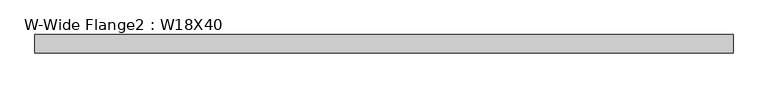
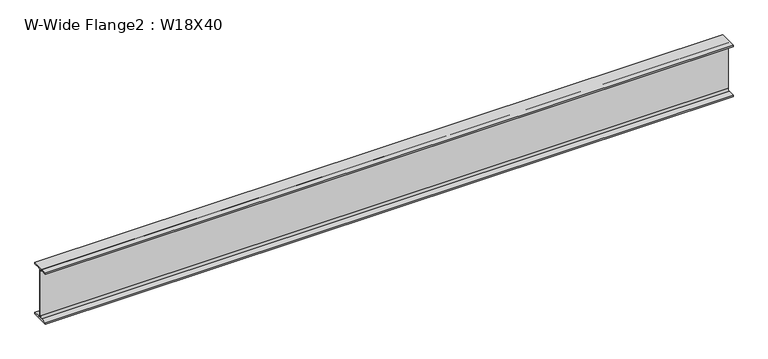
"""IFC4 building model written with IfcOpenShell, lengths in millimetres: beam geometry, W-Wide Flange2 : W18X40."""

import ifcopenshell
import ifcopenshell.guid

model = None  # the IFC model being written
_history = None  # IfcOwnerHistory: only IFC2X3 demands one
_inside = {}  # id of a spatial element -> (the spatial element, [elements in it])
_under = {}  # id of a project, library or spatial element -> (it, [spatial elements below it])
_declared = {}  # id of a project -> (the project, [libraries it declares])
_typed = {}  # id of a type object -> (the type object, [elements of that type])
_made_of = {}  # id of a material, layer set ... -> (it, [elements and type objects made of it])


def new_model(schema):
    """Start an empty IFC model of exactly this schema.

    Asked for "IFC4X3", IfcOpenShell would pick the latest addendum, in which some entities
    have other attributes; the version numbers below select the first issue.
    IFC2X3 requires an IfcOwnerHistory on every rooted entity: one is made here for all.
    """
    global model, _history
    if schema == "IFC4X3":
        model = ifcopenshell.file(schema_version=(4, 3, 0, 0))
    else:
        model = ifcopenshell.file(schema=schema)
    _inside.clear()
    _under.clear()
    _declared.clear()
    _typed.clear()
    _made_of.clear()
    _history = None
    if model.schema == "IFC2X3":
        org = make("IfcOrganization", Name="unknown")
        user = make(
            "IfcPersonAndOrganization",
            ThePerson=make("IfcPerson", FamilyName="unknown"),
            TheOrganization=org,
        )
        app = make(
            "IfcApplication",
            ApplicationDeveloper=org,
            Version="unknown",
            ApplicationFullName="unknown",
            ApplicationIdentifier="unknown",
        )
        _history = make(
            "IfcOwnerHistory",
            OwningUser=user,
            OwningApplication=app,
            ChangeAction="ADDED",
            CreationDate=0,
        )
    return model


def make(cls, **values):
    """One entity of the class cls with the attributes given. An attribute that is None is left unset."""
    return model.create_entity(
        cls, **{name: value for name, value in values.items() if value is not None}
    )


def rooted(cls, **values):
    """An entity with a GlobalId (a new one), such as an element, a storey or a relation."""
    return make(cls, GlobalId=ifcopenshell.guid.new(), OwnerHistory=_history, **values)


def si_unit(unit_type, name, prefix=None):
    """IfcSIUnit, for example si_unit("LENGTHUNIT", "METRE", prefix="MILLI")."""
    return make("IfcSIUnit", UnitType=unit_type, Prefix=prefix, Name=name)


def assignment(units):
    """IfcUnitAssignment: the units of a project."""
    return None if units is None else make("IfcUnitAssignment", Units=units)


def point(xyz):
    """IfcCartesianPoint."""
    return None if xyz is None else make("IfcCartesianPoint", Coordinates=xyz)


def direction(xyz):
    """IfcDirection."""
    return None if xyz is None else make("IfcDirection", DirectionRatios=xyz)


def frame(location, z_axis=None, x_axis=None):
    """IfcAxis2Placement3D, a coordinate frame: its origin and axes. An axis left out is left unset."""
    return make(
        "IfcAxis2Placement3D",
        Location=point(location),
        Axis=direction(z_axis),
        RefDirection=direction(x_axis),
    )


def frame_2d(location, x_axis=None):
    """IfcAxis2Placement2D, a coordinate frame in the plane: its origin and x axis."""
    return make(
        "IfcAxis2Placement2D", Location=point(location), RefDirection=direction(x_axis)
    )


def origin():
    """The frame at (0, 0, 0) with its axes left unset."""
    return frame((0.0, 0.0, 0.0))


def place(relative_to, where):
    """IfcLocalPlacement: puts the frame where relative to a parent placement (None: the world)."""
    return make(
        "IfcLocalPlacement", PlacementRelTo=relative_to, RelativePlacement=where
    )


def context(
    kind, dimensions, precision=None, world=None, true_north=None, identifier=None
):
    """IfcGeometricRepresentationContext, for example the 3D "Model" context."""
    return make(
        "IfcGeometricRepresentationContext",
        ContextIdentifier=identifier,
        ContextType=kind,
        CoordinateSpaceDimension=dimensions,
        Precision=precision,
        WorldCoordinateSystem=world,
        TrueNorth=true_north,
    )


def project(units=None, contexts=None):
    """IfcProject with its units and contexts."""
    return rooted(
        "IfcProject",
        Name="project",
        RepresentationContexts=contexts,
        UnitsInContext=assignment(units),
    )


def spatial(cls, under=None, at=None, **own):
    """A site, building, storey or space (cls), placed at a placement, below another one or the project."""
    s = rooted(cls, ObjectPlacement=at, **own)
    if under is not None:
        _under.setdefault(under.id(), (under, []))[1].append(s)
    return s


def polyline(points):
    """IfcPolyline through the points."""
    return make("IfcPolyline", Points=[point(p) for p in points])


def circle_curve(where, radius):
    """IfcCircle in the frame where."""
    return make("IfcCircle", Position=where, Radius=radius)


def trimmed(basis, trim1, trim2, sense, master):
    """IfcTrimmedCurve: the piece of a basis curve between two trims."""
    return make(
        "IfcTrimmedCurve",
        BasisCurve=basis,
        Trim1=trim1,
        Trim2=trim2,
        SenseAgreement=sense,
        MasterRepresentation=master,
    )


def segment(curve, same_sense, transition):
    """IfcCompositeCurveSegment."""
    return make(
        "IfcCompositeCurveSegment",
        Transition=transition,
        SameSense=same_sense,
        ParentCurve=curve,
    )


def composite_curve(segments, self_intersect=None):
    """IfcCompositeCurve: segments joined end to end."""
    return make("IfcCompositeCurve", Segments=segments, SelfIntersect=self_intersect)


def outline(outer, holes=None, kind="AREA"):
    """IfcArbitraryClosedProfileDef: a profile drawn as a closed curve; with holes, ...WithVoids."""
    if holes is None:
        return make("IfcArbitraryClosedProfileDef", ProfileType=kind, OuterCurve=outer)
    return make(
        "IfcArbitraryProfileDefWithVoids",
        ProfileType=kind,
        OuterCurve=outer,
        InnerCurves=holes,
    )


def extrude(swept, where, along, depth):
    """IfcExtrudedAreaSolid: the profile swept, set in the frame where, extruded along a direction by depth."""
    return make(
        "IfcExtrudedAreaSolid",
        SweptArea=swept,
        Position=where,
        ExtrudedDirection=direction(along),
        Depth=depth,
    )


def shape(context_of_items, identifier, shape_type, items):
    """IfcShapeRepresentation: the items that make up one representation, for example the "Body"."""
    return make(
        "IfcShapeRepresentation",
        ContextOfItems=context_of_items,
        RepresentationIdentifier=identifier,
        RepresentationType=shape_type,
        Items=items,
    )


def source(mapping_origin, context_of_items, identifier, shape_type, items):
    """IfcRepresentationMap: a shape defined once, which mapped items show again and again."""
    return make(
        "IfcRepresentationMap",
        MappingOrigin=mapping_origin,
        MappedRepresentation=shape(context_of_items, identifier, shape_type, items),
    )


def transform(
    local_origin,
    x_axis=None,
    y_axis=None,
    z_axis=None,
    scale=None,
    scale2=None,
    scale3=None,
    uniform=True,
):
    """IfcCartesianTransformationOperator3D, or its non-uniform kind. x_axis, y_axis, z_axis: its Axis1, 2, 3."""
    if uniform:
        return make(
            "IfcCartesianTransformationOperator3D",
            Axis1=direction(x_axis),
            Axis2=direction(y_axis),
            LocalOrigin=point(local_origin),
            Scale=scale,
            Axis3=direction(z_axis),
        )
    return make(
        "IfcCartesianTransformationOperator3DnonUniform",
        Axis1=direction(x_axis),
        Axis2=direction(y_axis),
        LocalOrigin=point(local_origin),
        Scale=scale,
        Axis3=direction(z_axis),
        Scale2=scale2,
        Scale3=scale3,
    )


def mapped(mapping_source, mapping_target):
    """IfcMappedItem: shows the shape of a source again, moved by a transform."""
    return make(
        "IfcMappedItem", MappingSource=mapping_source, MappingTarget=mapping_target
    )


def made_of(thing, what):
    """Note that an element or type object is made of a material, layer set ...; save() writes the relation."""
    if what is not None:
        _made_of.setdefault(what.id(), (what, []))[1].append(thing)
    return thing


def element(
    cls,
    number,
    at=None,
    inside=None,
    cuts=None,
    type_object=None,
    material=None,
    context=None,
    identifier="Body",
    shape_type=None,
    held_by="IfcProductDefinitionShape",
    body=None,
    shapes=None,
    **own,
):
    """One element of the class cls, such as IfcWall. Its Tag is "e" and its number.

    at: its placement. inside: the storey or other place that contains it. cuts: it is an
    opening in that element (IfcRelVoidsElement). A single representation is given by context,
    identifier, shape_type and body (its items); several are given by shapes. held_by: the class
    of the entity that holds the representations. save() writes the other relations.
    """
    e = rooted(cls, Tag="e%d" % number, ObjectPlacement=at, **own)
    if body is not None:
        shapes = [shape(context, identifier, shape_type, body)]
    if shapes is not None:
        e.Representation = make(held_by, Representations=shapes)
    if inside is not None:
        _inside.setdefault(inside.id(), (inside, []))[1].append(e)
    if cuts is not None:
        rooted(
            "IfcRelVoidsElement", RelatingBuildingElement=cuts, RelatedOpeningElement=e
        )
    if type_object is not None:
        _typed.setdefault(type_object.id(), (type_object, []))[1].append(e)
    return made_of(e, material)


def aggregate(whole, parts):
    """IfcRelAggregates: a whole, such as a stair, and the parts it consists of."""
    return rooted("IfcRelAggregates", RelatingObject=whole, RelatedObjects=parts)


def save(model, path):
    """Write the relations noted so far, then the file.

    IfcRelAggregates (storeys below a building ...), IfcRelContainedInSpatialStructure (elements
    in a storey), IfcRelDefinesByType, IfcRelAssociatesMaterial and IfcRelDeclares: one each for
    every whole, place, type object, material and project.
    """
    for whole, parts in _under.values():
        aggregate(whole, parts)
    for where, things in _inside.values():
        rooted(
            "IfcRelContainedInSpatialStructure",
            RelatedElements=things,
            RelatingStructure=where,
        )
    for kind, things in _typed.values():
        rooted("IfcRelDefinesByType", RelatedObjects=things, RelatingType=kind)
    for what, things in _made_of.values():
        rooted("IfcRelAssociatesMaterial", RelatedObjects=things, RelatingMaterial=what)
    for by, libraries in _declared.values():
        rooted("IfcRelDeclares", RelatingContext=by, RelatedDefinitions=libraries)
    model.write(path)


def w_wide_flange2_w18x40_a80abbf0(model_context):
    return source(origin(), model_context, "Body", "SweptSolid", [
        extrude(outline(composite_curve([segment(polyline([(76.454, -213.995), (76.454, -227.33), (-76.454, -227.33), (-76.454, -213.995), (-20.828, -213.995)]), True, "CONTINUOUS"), segment(trimmed(circle_curve(frame_2d((-20.828, -197.1675)), 16.8275), [point((-20.828, -213.995))], [point((-4.0005, -197.1675))], True, "CARTESIAN"), True, "CONTINUOUS"), segment(polyline([(-4.0005, -197.1675), (-4.0005, 197.1675)]), True, "CONTINUOUS"), segment(trimmed(circle_curve(frame_2d((-20.828, 197.1675)), 16.8275), [point((-4.0005, 197.1675))], [point((-20.828, 213.995))], True, "CARTESIAN"), True, "CONTINUOUS"), segment(polyline([(-20.828, 213.995), (-76.454, 213.995), (-76.454, 227.33), (76.454, 227.33), (76.454, 213.995), (20.828, 213.995)]), True, "CONTINUOUS"), segment(trimmed(circle_curve(frame_2d((20.828, 197.1675)), 16.8275), [point((20.828, 213.995))], [point((4.0005, 197.1675))], True, "CARTESIAN"), True, "CONTINUOUS"), segment(polyline([(4.0005, 197.1675), (4.0005, -197.1675)]), True, "CONTINUOUS"), segment(trimmed(circle_curve(frame_2d((20.828, -197.1675)), 16.8275), [point((4.0005, -197.1675))], [point((20.828, -213.995))], True, "CARTESIAN"), True, "CONTINUOUS"), segment(polyline([(20.828, -213.995), (76.454, -213.995)]), True, "CONTINUOUS")], self_intersect=False)), frame((-2876.153125, 0.0, 0.0), z_axis=(1.0, 0.0, 0.0), x_axis=(0.0, 1.0, 0.0)), (0.0, 0.0, 1.0), 5752.30625),
    ])


if __name__ == "__main__":
    model = new_model("IFC4")
    model_context = context("Model", 3, world=origin())
    ifc_project = project(units=[si_unit("LENGTHUNIT", "METRE", prefix="MILLI")], contexts=[model_context])
    site = spatial("IfcSite", under=ifc_project)
    building = spatial("IfcBuilding", under=site)
    placement = place(None, origin())
    w_wide_flange2_w18x40_shape = w_wide_flange2_w18x40_a80abbf0(model_context)
    element("IfcBeam", 1, ObjectType="W-Wide Flange2 : W18X40", at=placement, inside=building, context=model_context, shape_type="MappedRepresentation", body=[
        mapped(w_wide_flange2_w18x40_shape, transform((0.0, 0.0, 0.0), x_axis=(1.0, 0.0, 0.0), y_axis=(0.0, 1.0, 0.0), z_axis=(0.0, 0.0, 1.0))),
    ])
    save(model, "model.ifc")

# Revit data of these elements
# Type "W-Wide Flange2 : W18X40"
#   Assembly Code = "B10"
#   W = 40
#   Length [instance default] = 5' - 0"
#   bf = 0' - 6.02"
#   d = 1' - 5.9"
#   k = 0' - 1 3/16"
#   k2 = 0' - 0.6625"
#   tf = 0' - 0.525"
#   tw = 0' - 0.315"
#   A = 0.0819444 SF
#   Structural Material [instance default] = Steel ASTM A992
# Element 1 (IfcBeam, "W-Wide Flange2 : W18X40")
#   Materials on its faces: "Steel ASTM A992"
# Materials
#   "Steel ASTM A992": class "Metal", colour RGB 199 199 199, transparency 0, Description = "Structural steel 50ksi", Cost = 0
